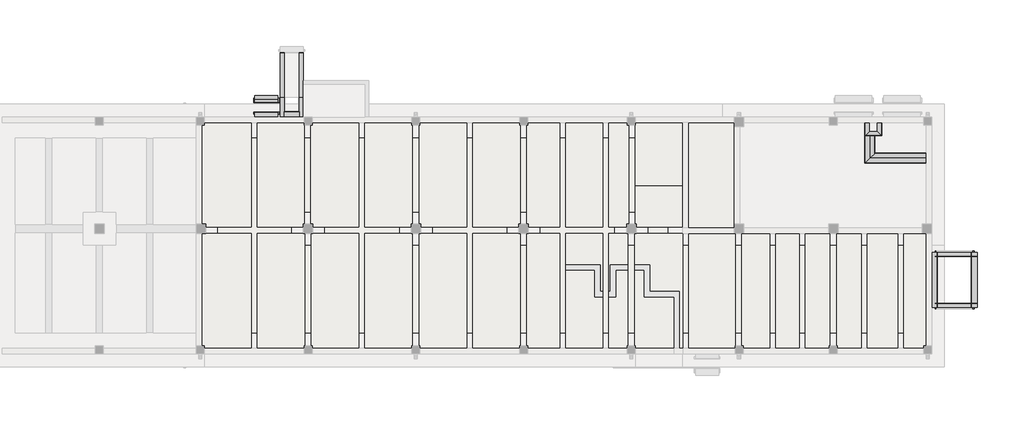
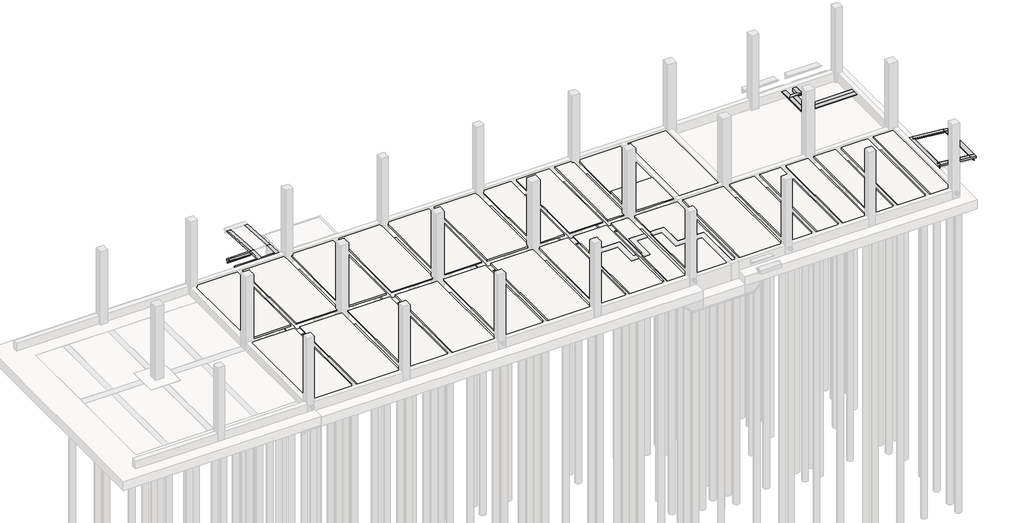
# One storey, part 2 of 7: 20 proxies, 4 slabs.
"""IFC4 building model written with IfcOpenShell, lengths in millimetres."""

from ifc_helpers import new_model, si_unit, frame, origin, place, context, project, spatial, polyline, outline, extrude, faceted_brep, element, save

model = new_model("IFC4")

# Units and contexts
model_context = context("Model", 3, world=origin())
ifc_project = project(units=[si_unit("LENGTHUNIT", "METRE", prefix="MILLI")], contexts=[model_context])

# Site, building, storey
site = spatial("IfcSite", under=ifc_project)
building = spatial("IfcBuilding", under=site)
storey = spatial("IfcBuildingStorey", under=building, Name="H.P.P", Elevation=4500.0)

# Proxies
placement = place(None, origin())
element("IfcBuildingElementProxy", 1, Name="H_SF_AR_B08_Ramp_T150_FrontEdge", ObjectType="H_SF_AR_B08_Ramp_T150_FrontEdge", at=placement, inside=storey, context=model_context, shape_type="Brep", body=[
    faceted_brep([(69312.0, -9750.0, 4500.0), (69312.0, -9750.0, 4650.0), (69700.0, -9750.0, 4650.0), (69699.3198779, -9750.0, 4649.3198779), (69562.2761194, -9750.0, 4512.2761194), (69550.0, -9750.0, 4500.0), (69312.0, -13850.0, 4650.0), (69312.0, -13850.0, 4500.0), (69550.0, -13850.0, 4500.0), (69562.2761194, -13850.0, 4512.2761194), (69699.3198779, -13850.0, 4649.3198779), (69700.0, -13850.0, 4650.0)], [[[0, 1, 2, 3, 4, 5]], [[6, 7, 8, 9, 10, 11]], [[1, 0, 7, 6]], [[8, 5, 4, 3, 2, 11, 10, 9]], [[0, 5, 8, 7]], [[2, 1, 6, 11]]]),
])
element("IfcBuildingElementProxy", 2, Name="H_SF_AR_B08_Ramp_T150_SideEdge", ObjectType="H_SF_AR_B08_Ramp_T150_SideEdge", at=placement, inside=storey, context=model_context, shape_type="Brep", body=[
    faceted_brep([(72700.0, -9750.0, 4198.5037314), (72700.0, -9750.0, 4349.2518657), (72700.0, -10050.0, 4349.2518657), (72700.0, -9900.7444215, 4199.2518657), (72700.0, -9900.0, 4198.5037314), (72692.5186568, -9750.0, 4199.2518657), (72423.0534826, -9750.0, 4226.1983831), (69562.2761194, -9750.0, 4512.2761194), (69699.3198779, -9750.0, 4649.3198779), (69700.0, -9750.0, 4649.2518657), (72250.0, -9750.0, 4394.2518657), (72256.3868159, -9750.0, 4393.6131841), (69699.3198779, -10050.0, 4649.3198779), (69700.0, -10050.0, 4649.2518657), (72250.0, -10050.0, 4394.2518657), (72255.5555556, -10050.0, 4393.6963101), (72256.3868159, -10050.0, 4393.6131841), (69562.2761194, -9900.0, 4512.2761194), (69626.5585541, -9900.0, 4505.847876), (72345.3173228, -9900.0, 4233.9719991), (72423.0534826, -9900.0, 4226.1983831), (72423.8847429, -9900.0, 4226.1152571), (72692.5186568, -9900.0, 4199.2518657)], [[[0, 1, 2, 3, 4]], [[1, 0, 5, 6, 7, 8, 9, 10, 11]], [[2, 1, 11, 10, 9, 8, 12, 13, 14, 15, 16]], [[4, 3, 2, 16, 15, 14, 13, 12, 17, 18, 19, 20, 21, 22]], [[0, 4, 22, 21, 20, 19, 18, 17, 7, 6, 5]], [[8, 7, 17, 12]]]),
    faceted_brep([(72700.0, -13850.0, 4349.2518657), (72700.0, -13850.0, 4198.5037314), (72700.0, -13700.0, 4198.5037314), (72700.0, -13699.2555785, 4199.2518657), (72700.0, -13550.0, 4349.2518657), (72256.3868159, -13850.0, 4393.6131841), (72250.0, -13850.0, 4394.2518657), (69700.0, -13850.0, 4649.2518657), (69699.3198779, -13850.0, 4649.3198779), (69562.2761194, -13850.0, 4512.2761194), (72423.0534826, -13850.0, 4226.1983831), (72692.5186568, -13850.0, 4199.2518657), (72256.3868159, -13550.0, 4393.6131841), (72255.5555556, -13550.0, 4393.6963101), (72250.0, -13550.0, 4394.2518657), (69700.0, -13550.0, 4649.2518657), (69699.3198779, -13550.0, 4649.3198779), (72692.5186568, -13700.0, 4199.2518657), (72423.8847429, -13700.0, 4226.1152571), (72423.0534826, -13700.0, 4226.1983831), (72345.3173228, -13700.0, 4233.9719991), (69626.5585541, -13700.0, 4505.847876), (69562.2761194, -13700.0, 4512.2761194)], [[[0, 1, 2, 3, 4]], [[1, 0, 5, 6, 7, 8, 9, 10, 11]], [[0, 4, 12, 13, 14, 15, 16, 8, 7, 6, 5]], [[4, 3, 2, 17, 18, 19, 20, 21, 22, 16, 15, 14, 13, 12]], [[2, 1, 11, 10, 9, 22, 21, 20, 19, 18, 17]], [[9, 8, 16, 22]]]),
])
element("IfcBuildingElementProxy", 3, Name="H_SF_AR_B08_Ramp_T150_FrontEdge(SLOPE)", ObjectType="H_SF_AR_B08_Ramp_T150_FrontEdge(SLOPE)", at=placement, inside=storey, context=model_context, shape_type="Brep", body=[
    faceted_brep([(72450.0, -13850.0, 4199.2518657), (72692.5186568, -13850.0, 4199.2518657), (72423.0534826, -13850.0, 4226.1983831), (72692.5186568, -9750.0, 4199.2518657), (72450.0, -9750.0, 4199.2518657), (72423.0534826, -9750.0, 4226.1983831), (72700.0, -13699.2555785, 4199.2518657), (72700.0, -9900.7444215, 4199.2518657), (72700.0, -10050.0, 4349.2518657), (72700.0, -13550.0, 4349.2518657), (72692.5186568, -9900.0, 4199.2518657), (72692.5186568, -13700.0, 4199.2518657), (72423.0534826, -13700.0, 4226.1983831), (72255.5555556, -13550.0, 4393.6963101), (72255.5555556, -10050.0, 4393.6963101), (72423.0534826, -9900.0, 4226.1983831)], [[[0, 1, 2]], [[3, 4, 5]], [[6, 7, 8, 9]], [[0, 4, 3, 10, 7, 6, 11, 1]], [[4, 0, 2, 12, 13, 14, 15, 5]], [[9, 8, 14, 13]], [[10, 15, 14, 8, 7]], [[15, 10, 3, 5]], [[12, 11, 6, 9, 13]], [[11, 12, 2, 1]]]),
])
element("IfcBuildingElementProxy", 4, Name="H_SF_AR_S18_Lean_T50_150X150", ObjectType="H_SF_AR_S18_Lean_T50_150X150", at=placement, inside=storey, context=model_context, shape_type="Brep", body=[
    faceted_brep([(69550.0, -13950.0, 4500.0), (69550.0, -13950.0, 4450.0), (69570.7106781, -13950.0, 4450.0), (69580.8773013, -13950.0, 4460.1666231), (69626.5585541, -13950.0, 4505.847876), (69562.2761194, -13950.0, 4512.2761194), (69550.0, -9650.0, 4450.0), (69550.0, -9650.0, 4500.0), (69562.2761194, -9650.0, 4512.2761194), (69626.5585541, -9650.0, 4505.847876), (69580.8773013, -9650.0, 4460.1666231), (69570.7106781, -9650.0, 4450.0), (69562.2761194, -13850.0, 4512.2761194), (69562.2761194, -13700.0, 4512.2761194), (69699.3198779, -13550.0, 4649.3198779), (69699.3198779, -13850.0, 4649.3198779), (69700.0, -13850.0, 4650.0), (69700.0, -9750.0, 4650.0), (69699.3198779, -9750.0, 4649.3198779), (69699.3198779, -10050.0, 4649.3198779), (69562.2761194, -9900.0, 4512.2761194), (69562.2761194, -9750.0, 4512.2761194), (69626.5585541, -9900.0, 4505.847876), (69720.7106781, -10003.0533515, 4600.0), (69720.7106781, -10050.0, 4600.0), (69717.9210597, -10050.0, 4597.2103816), (69717.9210597, -13550.0, 4597.2103816), (69720.7106781, -13550.0, 4600.0), (69720.7106781, -13596.9466485, 4600.0), (69626.5585541, -13700.0, 4505.847876), (69700.0, -13550.0, 4600.0), (69700.0, -13599.007438, 4600.0), (69700.0, -10050.0, 4600.0), (69700.0, -10000.992562, 4600.0), (69700.0, -13550.0, 4599.0024876), (69700.0, -10050.0, 4599.0024876), (69700.0, -10050.0, 4649.2518657), (69700.0, -9750.0, 4649.2518657), (69700.0, -13850.0, 4649.2518657), (69700.0, -13550.0, 4649.2518657)], [[[0, 1, 2, 3, 4, 5]], [[6, 7, 8, 9, 10, 11]], [[7, 0, 5, 12, 13, 14, 15, 16, 17, 18, 19, 20, 21, 8]], [[1, 0, 7, 6]], [[2, 1, 6, 11]], [[2, 11, 10, 9, 22, 23, 24, 25, 26, 27, 28, 29, 4, 3]], [[27, 30, 31, 28]], [[32, 24, 23, 33]], [[34, 35, 32, 33, 36, 37, 17, 16, 38, 39, 31, 30]], [[35, 34, 26, 25]], [[34, 30, 27, 26]], [[32, 35, 25, 24]], [[36, 19, 18, 37]], [[19, 36, 33, 23, 22, 20]], [[14, 39, 38, 15]], [[39, 14, 13, 29, 28, 31]], [[16, 15, 38]], [[5, 4, 29, 13, 12]], [[18, 17, 37]], [[9, 8, 21, 20, 22]]]),
])
element("IfcBuildingElementProxy", 5, Name="H_SF_AR_S18_Lean_T50_200X200", ObjectType="H_SF_AR_S18_Lean_T50_200X200", at=placement, inside=storey, context=model_context, shape_type="Brep", body=[
    faceted_brep([(72450.0, -9650.0, 4200.0), (72450.0, -9650.0, 4150.0), (72429.2893219, -9650.0, 4150.0), (72401.1499651, -9650.0, 4178.1393567), (72345.3173228, -9650.0, 4233.9719991), (72423.8847429, -9650.0, 4226.1152571), (72450.0, -13950.0, 4150.0), (72450.0, -13950.0, 4200.0), (72423.8847429, -13950.0, 4226.1152571), (72345.3173228, -13950.0, 4233.9719991), (72401.1499651, -13950.0, 4178.1393567), (72429.2893219, -13950.0, 4150.0), (72423.8847429, -9900.0, 4226.1152571), (72256.3868159, -10050.0, 4393.6131841), (72256.3868159, -9750.0, 4393.6131841), (72250.0, -9750.0, 4400.0), (72250.0, -13850.0, 4400.0), (72256.3868159, -13850.0, 4393.6131841), (72256.3868159, -13550.0, 4393.6131841), (72423.8847429, -13700.0, 4226.1152571), (72345.3173228, -13700.0, 4233.9719991), (72229.2893219, -13596.0930416, 4350.0), (72229.2893219, -13550.0, 4350.0), (72229.2893219, -10050.0, 4350.0), (72229.2893219, -10003.9069584, 4350.0), (72345.3173228, -9900.0, 4233.9719991), (72250.0, -13594.0322521, 4350.0), (72250.0, -13550.0, 4350.0), (72250.0, -10050.0, 4350.0), (72250.0, -10005.9677479, 4350.0), (72250.0, -9750.0, 4394.2518657), (72250.0, -10050.0, 4394.2518657), (72250.0, -13550.0, 4394.2518657), (72250.0, -13850.0, 4394.2518657)], [[[0, 1, 2, 3, 4, 5]], [[6, 7, 8, 9, 10, 11]], [[7, 0, 5, 12, 13, 14, 15, 16, 17, 18, 19, 8]], [[1, 0, 7, 6]], [[2, 1, 6, 11]], [[2, 11, 10, 9, 20, 21, 22, 23, 24, 25, 4, 3]], [[24, 23, 22, 21, 26, 27, 28, 29]], [[16, 15, 30, 31, 29, 28, 27, 26, 32, 33]], [[13, 31, 30, 14]], [[31, 13, 12, 25, 24, 29]], [[32, 18, 17, 33]], [[18, 32, 26, 21, 20, 19]], [[17, 16, 33]], [[9, 8, 19, 20]], [[15, 14, 30]], [[5, 4, 25, 12]]]),
])
element("IfcBuildingElementProxy", 6, Name="H_SF_AR_S18_Lean_T50_150X150", ObjectType="H_SF_AR_S18_Lean_T50_150X150", at=placement, inside=storey, context=model_context, shape_type="Brep", body=[
    faceted_brep([(72401.1499651, -13550.0, 4379.1368692), (72401.1499651, -13700.0, 4228.3887349), (72401.1499651, -13700.0, 4178.1393567), (72401.1499651, -13679.2893219, 4178.1393567), (72401.1499651, -13529.2893219, 4328.8874911), (72401.1499651, -13550.0, 4328.8874911), (69580.8773013, -13550.0, 4661.1641356), (69580.8773013, -13550.0, 4610.9147575), (69580.8773013, -13529.2893219, 4610.9147575), (69580.8773013, -13679.2893219, 4460.1666231), (69580.8773013, -13700.0, 4460.1666231), (69580.8773013, -13700.0, 4510.4160012)], [[[0, 1, 2, 3, 4, 5]], [[6, 7, 8, 9, 10, 11]], [[1, 0, 6, 11]], [[2, 1, 11, 10]], [[3, 2, 10, 9]], [[4, 3, 9, 8]], [[5, 4, 8, 7]], [[0, 5, 7, 6]]]),
])
element("IfcBuildingElementProxy", 7, Name="H_SF_AR_S18_Lean_T50_150X150", ObjectType="H_SF_AR_S18_Lean_T50_150X150", at=placement, inside=storey, context=model_context, shape_type="Brep", body=[
    faceted_brep([(69580.8773013, -10050.0, 4661.1641356), (69580.8773013, -9900.0, 4510.4160012), (69580.8773013, -9900.0, 4460.1666231), (69580.8773013, -9920.7106781, 4460.1666231), (69580.8773013, -10070.7106781, 4610.9147575), (69580.8773013, -10050.0, 4610.9147575), (72401.1499651, -10050.0, 4379.1368692), (72401.1499651, -10050.0, 4328.8874911), (72401.1499651, -10070.7106781, 4328.8874911), (72401.1499651, -9920.7106781, 4178.1393567), (72401.1499651, -9900.0, 4178.1393567), (72401.1499651, -9900.0, 4228.3887349)], [[[0, 1, 2, 3, 4, 5]], [[6, 7, 8, 9, 10, 11]], [[1, 0, 6, 11]], [[2, 1, 11, 10]], [[3, 2, 10, 9]], [[4, 3, 9, 8]], [[5, 4, 8, 7]], [[0, 5, 7, 6]]]),
])
element("IfcBuildingElementProxy", 8, Name="H_SF_AR_B08_Stoop_T150_FrontEdge", ObjectType="H_SF_AR_B08_Stoop_T150_FrontEdge", at=placement, inside=storey, context=model_context, shape_type="SweptSolid", body=[
    extrude(outline(polyline([(312.0000074, 4480.0), (312.0000074, 4630.0), (662.0000074, 4630.0), (512.0000074, 4480.0), (312.0000074, 4480.0)])), frame((19050.0, 0.0, 0.0), z_axis=(1.0, 0.0, 0.0), x_axis=(0.0, 1.0, 0.0)), (0.0, 0.0, 1.0), 1700.0),
])
element("IfcBuildingElementProxy", 9, Name="H_SF_AR_B08_Stoop_T150_FrontEdge_500x300", ObjectType="H_SF_AR_B08_Stoop_T150_FrontEdge_500x300", at=placement, inside=storey, context=model_context, shape_type="SweptSolid", body=[
    extrude(outline(polyline([(1700.0, 4330.0), (1400.0, 4630.0), (1600.0, 4630.0), (1600.0, 4515.0), (1900.0, 4515.0), (1900.0, 4330.0), (1700.0, 4330.0)])), frame((19050.0, 0.0, 0.0), z_axis=(1.0, 0.0, 0.0), x_axis=(0.0, 1.0, 0.0)), (0.0, 0.0, 1.0), 1700.0),
])
element("IfcBuildingElementProxy", 10, Name="H_SF_AR_S18_Lean_T50_300X300", ObjectType="H_SF_AR_S18_Lean_T50_300X300", at=placement, inside=storey, context=model_context, shape_type="SweptSolid", body=[
    extrude(outline(polyline([(1700.0, 4330.0), (1700.0, 4280.0), (1679.2893219, 4280.0), (1379.2893219, 4580.0), (1400.0, 4580.0), (1400.0, 4630.0), (1700.0, 4330.0)])), frame((18950.0, 0.0, 0.0), z_axis=(1.0, 0.0, 0.0), x_axis=(0.0, 1.0, 0.0)), (0.0, 0.0, 1.0), 1900.0),
])
element("IfcBuildingElementProxy", 11, Name="H_SF_AR_S18_Lean_T50_150X150", ObjectType="H_SF_AR_S18_Lean_T50_150X150", at=placement, inside=storey, context=model_context, shape_type="SweptSolid", body=[
    extrude(outline(polyline([(512.0000074, 4430.0), (512.0000074, 4480.0), (662.0000074, 4630.0), (662.0000074, 4580.0), (682.7106855, 4580.0), (532.7106855, 4430.0), (512.0000074, 4430.0)])), frame((18950.0, 0.0, 0.0), z_axis=(1.0, 0.0, 0.0), x_axis=(0.0, 1.0, 0.0)), (0.0, 0.0, 1.0), 1900.0),
])
element("IfcBuildingElementProxy", 12, Name="H_SF_AR_B08_Ramp_T150_FrontEdge", ObjectType="H_SF_AR_B08_Ramp_T150_FrontEdge", at=placement, inside=storey, context=model_context, shape_type="Brep", body=[
    faceted_brep([(21088.0, 312.0, 4450.0), (22488.0, 312.0, 4450.0), (22338.0, 312.0, 4600.0), (21238.0, 312.0, 4600.0), (22338.0, 700.0, 4600.0), (21238.0, 700.0, 4600.0), (22488.0, 550.0, 4450.0), (21088.0, 550.0, 4450.0)], [[[0, 1, 2, 3]], [[3, 2, 4, 5]], [[5, 4, 6, 7]], [[1, 0, 7, 6]], [[0, 3, 5, 7]], [[2, 1, 6, 4]]]),
])
element("IfcBuildingElementProxy", 13, Name="H_SF_AR_B08_Ramp_T150_SideEdge", ObjectType="H_SF_AR_B08_Ramp_T150_SideEdge", at=placement, inside=storey, context=model_context, shape_type="Brep", body=[
    faceted_brep([(20938.0, 1800.0, 4600.0), (21238.0, 1800.0, 4600.0), (21237.6670362, 1800.0, 4599.6670362), (21088.0, 1800.0, 4450.0), (20938.0, 1800.0, 4450.0), (20938.0, 1800.0, 4599.6670362), (20938.0, 312.0, 4600.0), (20938.0, 312.0, 4450.0), (21088.0, 312.0, 4450.0), (21238.0, 312.0, 4600.0), (21238.0, 700.0, 4600.0), (21088.0, 550.0, 4450.0)], [[[0, 1, 2, 3, 4, 5]], [[6, 7, 8, 9]], [[7, 6, 0, 5, 4]], [[1, 0, 6, 9, 10]], [[9, 8, 11, 3, 2, 1, 10]], [[4, 3, 11, 8, 7]]]),
    faceted_brep([(20938.0, 1800.0, 4599.6670362), (20938.0, 1800.0, 4449.3340724), (21088.0, 1800.0, 4449.3340724), (21238.0, 1800.0, 4599.6670362), (20938.0, 5100.0, 4379.6670362), (20938.0, 5260.3575388, 4219.3094974), (20938.0, 5261.0710326, 4218.5960036), (20938.0, 5185.3095918, 4223.6467663), (21238.0, 5100.0, 4379.6670362), (21088.0, 5185.3095918, 4223.6467663), (21088.0, 5261.0710326, 4218.5960036)], [[[0, 1, 2, 3]], [[1, 0, 4, 5, 6, 7]], [[0, 3, 8, 4]], [[3, 2, 9, 10, 8]], [[2, 1, 7, 6, 10, 9]], [[6, 5, 4, 8, 10]]]),
    faceted_brep([(22638.0, 1800.0, 4449.3340724), (22638.0, 1800.0, 4599.6670362), (22338.0, 1800.0, 4599.6670362), (22488.0, 1800.0, 4449.3340724), (22638.0, 5185.3095918, 4223.6467663), (22638.0, 5261.0710326, 4218.5960036), (22638.0, 5260.3575388, 4219.3094974), (22638.0, 5100.0, 4379.6670362), (22338.0, 5100.0, 4379.6670362), (22488.0, 5261.0710326, 4218.5960036), (22488.0, 5185.3095918, 4223.6467663)], [[[0, 1, 2, 3]], [[1, 0, 4, 5, 6, 7]], [[2, 1, 7, 8]], [[3, 2, 8, 9, 10]], [[0, 3, 10, 9, 5, 4]], [[7, 6, 5, 9, 8]]]),
    faceted_brep([(22638.0, 312.0, 4450.0), (22638.0, 312.0, 4600.0), (22338.0, 312.0, 4600.0), (22488.0, 312.0, 4450.0), (22338.0, 1800.0, 4600.0), (22638.0, 1800.0, 4600.0), (22638.0, 1800.0, 4599.6670362), (22638.0, 1800.0, 4450.0), (22488.0, 1800.0, 4450.0), (22338.3329638, 1800.0, 4599.6670362), (22338.0, 700.0, 4600.0), (22488.0, 550.0, 4450.0)], [[[0, 1, 2, 3]], [[4, 5, 6, 7, 8, 9]], [[1, 0, 7, 6, 5]], [[2, 1, 5, 4, 10]], [[3, 2, 10, 4, 9, 8, 11]], [[0, 3, 11, 8, 7]]]),
])
element("IfcBuildingElementProxy", 14, Name="H_SF_AR_S18_Lean_T50_150X150", ObjectType="H_SF_AR_S18_Lean_T50_150X150", at=placement, inside=storey, context=model_context, shape_type="Brep", body=[
    faceted_brep([(22338.0, 700.0, 4600.0), (22488.0, 550.0, 4450.0), (22488.0, 550.0, 4400.0), (22467.2893219, 570.7106781, 4400.0), (22317.2893219, 720.7106781, 4550.0), (22338.0, 700.0, 4550.0), (21088.0, 550.0, 4450.0), (21238.0, 700.0, 4600.0), (21238.0, 700.0, 4550.0), (21258.7106781, 720.7106781, 4550.0), (21108.7106781, 570.7106781, 4400.0), (21088.0, 550.0, 4400.0)], [[[0, 1, 2, 3, 4, 5]], [[6, 7, 8, 9, 10, 11]], [[1, 0, 7, 6]], [[2, 1, 6, 11]], [[3, 2, 11, 10]], [[4, 3, 10, 9]], [[5, 4, 9, 8]], [[0, 5, 8, 7]]]),
])
element("IfcBuildingElementProxy", 15, Name="H_SF_AR_S17_SOG Edge_350x150", ObjectType="H_SF_AR_S17_SOG Edge_350x150", at=placement, inside=storey, context=model_context, shape_type="Brep", body=[
    faceted_brep([(64707.0, -2743.0, 4500.0), (64707.0, -2743.0, 4650.0), (64707.0, -1062.0, 4650.0), (64707.0, -912.0, 4500.0), (65057.0, -2393.0, 4650.0), (64907.0, -2543.0, 4500.0), (64907.0, -982.7106781, 4500.0), (64907.0, -912.0, 4500.0), (65057.0, -1062.0, 4650.0), (68888.0, -2743.0, 4650.0), (68888.0, -2743.0, 4500.0), (68888.0, -2543.0, 4500.0), (68888.0, -2393.0, 4650.0)], [[[0, 1, 2, 3]], [[4, 5, 6, 7, 8]], [[5, 0, 3, 7, 6]], [[1, 4, 8, 2]], [[9, 10, 11, 12]], [[1, 0, 10, 9]], [[4, 1, 9, 12]], [[5, 4, 12, 11]], [[0, 5, 11, 10]], [[3, 2, 8, 7]]]),
])
element("IfcBuildingElementProxy", 16, Name="H_SF_AR_S17_SOG Edge_350x150", ObjectType="H_SF_AR_S17_SOG Edge_350x150", at=placement, inside=storey, context=model_context, shape_type="Brep", body=[
    faceted_brep([(64707.0, -2743.0, 4650.0), (64707.0, -2743.0, 4500.0), (64707.0, -912.0, 4500.0), (64707.0, -1062.0, 4650.0), (64357.0, -3093.0, 4650.0), (64357.0, -1062.0, 4650.0), (64507.0, -2943.0, 4500.0), (64507.0, -912.0, 4500.0), (64507.0, -982.7106781, 4500.0), (68888.0, -2743.0, 4500.0), (68888.0, -2743.0, 4650.0), (68888.0, -3093.0, 4650.0), (68888.0, -2943.0, 4500.0)], [[[0, 1, 2, 3]], [[4, 0, 3, 5]], [[6, 4, 5, 7, 8]], [[1, 6, 8, 7, 2]], [[9, 10, 11, 12]], [[1, 0, 10, 9]], [[0, 4, 11, 10]], [[4, 6, 12, 11]], [[6, 1, 9, 12]], [[3, 2, 7, 5]]]),
])
element("IfcBuildingElementProxy", 17, Name="H_SF_AR_S17_SOG Edge_300x300", ObjectType="H_SF_AR_S17_SOG Edge_300x300", at=placement, inside=storey, context=model_context, shape_type="Brep", body=[
    faceted_brep([(64657.0, -112.0, 4350.0), (64357.0, -112.0, 4650.0), (64657.0, -112.0, 4650.0), (64357.0, -1062.0, 4650.0), (64657.0, -762.0, 4650.0), (64657.0, -762.0, 4350.0), (64507.0, -912.0, 4500.0), (65257.0, -762.0, 4350.0), (65557.0, -1062.0, 4650.0), (65057.0, -1062.0, 4650.0), (64707.0, -1062.0, 4650.0), (65257.0, -762.0, 4650.0), (65557.0, -112.0, 4650.0), (65257.0, -112.0, 4350.0), (65257.0, -112.0, 4650.0)], [[[0, 1, 2]], [[1, 3, 4, 2]], [[1, 0, 5, 6, 3]], [[3, 6, 5, 7, 8, 9, 10]], [[3, 10, 9, 8, 11, 4]], [[12, 13, 14]], [[8, 7, 13, 12]], [[8, 12, 14, 11]], [[7, 11, 14, 13]], [[11, 7, 5, 4]], [[4, 5, 0, 2]]]),
])
element("IfcBuildingElementProxy", 18, Name="H_SF_AR_S18_Lean_T50_150X150", ObjectType="H_SF_AR_S18_Lean_T50_150X150", at=placement, inside=storey, context=model_context, shape_type="Brep", body=[
    faceted_brep([(64357.0, -3093.0, 4650.0), (64507.0, -2943.0, 4500.0), (64507.0, -982.7106781, 4500.0), (64407.0, -1082.7106781, 4600.0), (64407.0, -1062.0, 4600.0), (64357.0, -1062.0, 4650.0), (64507.0, -2943.0, 4450.0), (64507.0, -932.7106781, 4450.0), (64486.2893219, -2963.7106781, 4450.0), (64486.2893219, -932.7106781, 4450.0), (64336.2893219, -3113.7106781, 4600.0), (64336.2893219, -1082.7106781, 4600.0), (64357.0, -3093.0, 4600.0), (64357.0, -1082.7106781, 4600.0), (64357.0, -1062.0, 4600.0), (68900.0, -2943.0, 4500.0), (68900.0, -3093.0, 4650.0), (68900.0, -3093.0, 4600.0), (68900.0, -3113.7106781, 4600.0), (68900.0, -2963.7106781, 4450.0), (68900.0, -2943.0, 4450.0)], [[[0, 1, 2, 3, 4, 5]], [[1, 6, 7, 2]], [[6, 8, 9, 7]], [[8, 10, 11, 9]], [[10, 12, 13, 11]], [[12, 0, 5, 14, 13]], [[15, 16, 17, 18, 19, 20]], [[1, 0, 16, 15]], [[6, 1, 15, 20]], [[8, 6, 20, 19]], [[10, 8, 19, 18]], [[12, 10, 18, 17]], [[0, 12, 17, 16]], [[13, 3, 2, 7, 9, 11]], [[3, 13, 14, 4]], [[4, 14, 5]]]),
])
element("IfcBuildingElementProxy", 19, Name="H_SF_AR_S18_Lean_T50_150X150", ObjectType="H_SF_AR_S18_Lean_T50_150X150", at=placement, inside=storey, context=model_context, shape_type="Brep", body=[
    faceted_brep([(64907.0, -2543.0, 4500.0), (65057.0, -2393.0, 4650.0), (65057.0, -1062.0, 4650.0), (65007.0, -1062.0, 4600.0), (65007.0, -1082.7106781, 4600.0), (64907.0, -982.7106781, 4500.0), (64907.0, -2543.0, 4450.0), (64907.0, -932.7106781, 4450.0), (64927.7106781, -2522.2893219, 4450.0), (64927.7106781, -932.7106781, 4450.0), (65077.7106781, -2372.2893219, 4600.0), (65077.7106781, -1082.7106781, 4600.0), (65057.0, -2393.0, 4600.0), (65057.0, -1082.7106781, 4600.0), (65057.0, -1062.0, 4600.0), (68900.0, -2393.0, 4650.0), (68900.0, -2543.0, 4500.0), (68900.0, -2543.0, 4450.0), (68900.0, -2522.2893219, 4450.0), (68900.0, -2372.2893219, 4600.0), (68900.0, -2393.0, 4600.0)], [[[0, 1, 2, 3, 4, 5]], [[6, 0, 5, 7]], [[8, 6, 7, 9]], [[10, 8, 9, 11]], [[12, 10, 11, 13]], [[1, 12, 13, 14, 2]], [[15, 16, 17, 18, 19, 20]], [[1, 0, 16, 15]], [[0, 6, 17, 16]], [[6, 8, 18, 17]], [[8, 10, 19, 18]], [[10, 12, 20, 19]], [[12, 1, 15, 20]], [[4, 13, 11, 9, 7, 5]], [[13, 4, 3, 14]], [[14, 3, 2]]]),
])
element("IfcBuildingElementProxy", 20, Name="H_SF_AR_S18_Lean_T50_300X300", ObjectType="H_SF_AR_S18_Lean_T50_300X300", at=placement, inside=storey, context=model_context, shape_type="Brep", body=[
    faceted_brep([(64357.0, -100.0, 4650.0), (64657.0, -100.0, 4350.0), (64657.0, -100.0, 4300.0), (64636.2893219, -100.0, 4300.0), (64336.2893219, -100.0, 4600.0), (64357.0, -100.0, 4600.0), (64357.0, -1062.0, 4650.0), (64407.0, -1062.0, 4600.0), (64407.0, -1082.7106781, 4600.0), (64507.0, -982.7106781, 4500.0), (64507.0, -912.0, 4500.0), (64657.0, -762.0, 4350.0), (64657.0, -762.0, 4300.0), (64636.2893219, -782.7106781, 4300.0), (64486.2893219, -932.7106781, 4450.0), (64336.2893219, -1082.7106781, 4600.0), (64357.0, -1062.0, 4600.0), (65557.0, -1062.0, 4650.0), (65257.0, -762.0, 4350.0), (64707.0, -912.0, 4500.0), (64907.0, -912.0, 4500.0), (65057.0, -1062.0, 4650.0), (65257.0, -762.0, 4300.0), (65277.7106781, -782.7106781, 4300.0), (65577.7106781, -1082.7106781, 4600.0), (65077.7106781, -1082.7106781, 4600.0), (65057.0, -1082.7106781, 4600.0), (65007.0, -1082.7106781, 4600.0), (64907.0, -982.7106781, 4500.0), (64357.0, -1082.7106781, 4600.0), (65557.0, -1062.0, 4600.0), (65057.0, -1062.0, 4600.0), (65007.0, -1062.0, 4600.0), (65257.0, -100.0, 4350.0), (65557.0, -100.0, 4650.0), (65557.0, -100.0, 4600.0), (65577.7106781, -100.0, 4600.0), (65277.7106781, -100.0, 4300.0), (65257.0, -100.0, 4300.0)], [[[0, 1, 2, 3, 4, 5]], [[1, 0, 6, 7, 8, 9, 10, 11]], [[11, 12, 2, 1]], [[12, 13, 3, 2]], [[13, 14, 15, 4, 3]], [[15, 16, 5, 4]], [[16, 6, 0, 5]], [[17, 18, 11, 10, 19, 20, 21]], [[12, 11, 18, 22]], [[13, 12, 22, 23]], [[15, 14, 13, 23, 24, 25, 26, 27, 28, 9, 8, 29]], [[16, 15, 29, 8, 7]], [[24, 30, 31, 32, 27, 26, 25]], [[6, 16, 7]], [[30, 17, 21, 32, 31]], [[33, 34, 35, 36, 37, 38]], [[18, 17, 34, 33]], [[22, 18, 33, 38]], [[23, 22, 38, 37]], [[24, 23, 37, 36]], [[30, 24, 36, 35]], [[17, 30, 35, 34]], [[10, 9, 28, 20, 19]], [[20, 28, 27, 32, 21]]]),
])

# Slabs
element("IfcSlab", 21, ObjectType="H_FL_AR_B07_Ground Insulation_T110", at=placement, inside=storey, context=model_context, shape_type="SweptSolid", body=[
    extrude(outline(polyline([(15100.0, -8350.0), (18775.0, -8350.0), (18775.0, -16900.0), (15300.0, -16900.0), (15300.0, -16700.0), (15100.0, -16700.0), (15100.0, -8350.0)])), frame((0.0, 0.0, 4540.0), z_axis=(0.0, 0.0, 1.0), x_axis=(1.0, 0.0, 0.0)), (0.0, 0.0, 1.0), 110.0),
    extrude(outline(polyline([(15400.0000001, -7850.0), (15400.0000001, -7650.0), (15100.0, -7650.0), (15100.0, -300.0), (15300.0, -300.0), (15300.0, -100.0), (18775.0, -100.0), (18775.0, -7850.0), (15400.0000001, -7850.0)])), frame((0.0, 0.0, 4540.0), z_axis=(0.0, 0.0, 1.0), x_axis=(1.0, 0.0, 0.0)), (0.0, 0.0, 1.0), 110.0),
    extrude(outline(polyline([(22750.0, -8350.0), (22750.0, -16700.0), (22700.0, -16700.0), (22700.0, -16900.0), (19225.0, -16900.0), (19225.0, -8350.0), (22750.0, -8350.0)])), frame((0.0, 0.0, 4540.0), z_axis=(0.0, 0.0, 1.0), x_axis=(1.0, 0.0, 0.0)), (0.0, 0.0, 1.0), 110.0),
    extrude(outline(polyline([(22650.0000003, -7850.0), (19225.0, -7850.0), (19225.0, -100.0), (22700.0, -100.0), (22700.0, -7650.0), (22650.0000003, -7650.0), (22650.0000003, -7850.0)])), frame((0.0, 0.0, 4540.0), z_axis=(0.0, 0.0, 1.0), x_axis=(1.0, 0.0, 0.0)), (0.0, 0.0, 1.0), 110.0),
    extrude(outline(polyline([(23250.0, -8350.0), (26775.0, -8350.0), (26775.0, -16900.0), (23300.0, -16900.0), (23300.0, -16700.0), (23250.0, -16700.0), (23250.0, -8350.0)])), frame((0.0, 0.0, 4540.0), z_axis=(0.0, 0.0, 1.0), x_axis=(1.0, 0.0, 0.0)), (0.0, 0.0, 1.0), 110.0),
    extrude(outline(polyline([(23350.0000003, -7850.0), (23350.0000003, -7650.0), (23200.0, -7650.0), (23200.0, -300.0), (23300.0, -300.0), (23300.0, -100.0), (26775.0, -100.0), (26775.0, -7850.0), (23350.0000003, -7850.0)])), frame((0.0, 0.0, 4540.0), z_axis=(0.0, 0.0, 1.0), x_axis=(1.0, 0.0, 0.0)), (0.0, 0.0, 1.0), 110.0),
    extrude(outline(polyline([(30750.0, -8350.0), (30750.0, -16700.0), (30700.0, -16700.0), (30700.0, -16900.0), (27225.0, -16900.0), (27225.0, -8350.0), (30750.0, -8350.0)])), frame((0.0, 0.0, 4540.0), z_axis=(0.0, 0.0, 1.0), x_axis=(1.0, 0.0, 0.0)), (0.0, 0.0, 1.0), 110.0),
    extrude(outline(polyline([(30650.0000002, -7850.0), (27225.0, -7850.0), (27225.0, -100.0), (30700.0, -100.0), (30700.0, -300.0), (30750.0, -300.0), (30750.0, -7650.0), (30650.0000002, -7650.0), (30650.0000002, -7850.0)])), frame((0.0, 0.0, 4540.0), z_axis=(0.0, 0.0, 1.0), x_axis=(1.0, 0.0, 0.0)), (0.0, 0.0, 1.0), 110.0),
    extrude(outline(polyline([(31250.0, -8350.0), (34775.0, -8350.0), (34775.0, -16900.0), (31300.0, -16900.0), (31300.0, -16700.0), (31250.0, -16700.0), (31250.0, -8350.0)])), frame((0.0, 0.0, 4540.0), z_axis=(0.0, 0.0, 1.0), x_axis=(1.0, 0.0, 0.0)), (0.0, 0.0, 1.0), 110.0),
    extrude(outline(polyline([(31350.0000002, -7850.0), (31350.0000002, -7650.0), (31250.0, -7650.0), (31250.0, -300.0), (31300.0, -300.0), (31300.0, -100.0), (34775.0, -100.0), (34775.0, -7850.0), (31350.0000002, -7850.0)])), frame((0.0, 0.0, 4540.0), z_axis=(0.0, 0.0, 1.0), x_axis=(1.0, 0.0, 0.0)), (0.0, 0.0, 1.0), 110.0),
    extrude(outline(polyline([(38750.0, -8350.0), (38750.0, -16700.0), (38700.0, -16700.0), (38700.0, -16900.0), (35225.0, -16900.0), (35225.0, -8350.0), (38750.0, -8350.0)])), frame((0.0, 0.0, 4540.0), z_axis=(0.0, 0.0, 1.0), x_axis=(1.0, 0.0, 0.0)), (0.0, 0.0, 1.0), 110.0),
    extrude(outline(polyline([(38650.0000001, -7850.0), (35225.0, -7850.0), (35225.0, -100.0), (38700.0, -100.0), (38700.0, -300.0), (38750.0, -300.0), (38750.0, -7650.0), (38650.0000001, -7650.0), (38650.0000001, -7850.0)])), frame((0.0, 0.0, 4540.0), z_axis=(0.0, 0.0, 1.0), x_axis=(1.0, 0.0, 0.0)), (0.0, 0.0, 1.0), 110.0),
    extrude(outline(polyline([(39250.0, -8350.0), (41675.0, -8350.0), (41675.0, -16900.0), (39300.0, -16900.0), (39300.0, -16700.0), (39250.0, -16700.0), (39250.0, -8350.0)])), frame((0.0, 0.0, 4540.0), z_axis=(0.0, 0.0, 1.0), x_axis=(1.0, 0.0, 0.0)), (0.0, 0.0, 1.0), 110.0),
    extrude(outline(polyline([(39350.0000001, -7850.0), (39350.0000001, -7650.0), (39250.0, -7650.0), (39250.0, -300.0), (39300.0, -300.0), (39300.0, -100.0), (41675.0, -100.0), (41675.0, -7850.0), (39350.0000001, -7850.0)])), frame((0.0, 0.0, 4540.0), z_axis=(0.0, 0.0, 1.0), x_axis=(1.0, 0.0, 0.0)), (0.0, 0.0, 1.0), 110.0),
    extrude(outline(polyline([(44875.0, -100.0), (44875.0, -7850.0), (42125.0, -7850.0), (42125.0, -100.0), (44875.0, -100.0)])), frame((0.0, 0.0, 4540.0), z_axis=(0.0, 0.0, 1.0), x_axis=(1.0, 0.0, 0.0)), (0.0, 0.0, 1.0), 110.0),
    extrude(outline(polyline([(44875.0, -8350.0), (44875.0, -12675.0), (44675.0, -12675.0), (44675.0, -10675.0), (42125.0, -10675.0), (42125.0, -8350.0), (44875.0, -8350.0)])), frame((0.0, 0.0, 4540.0), z_axis=(0.0, 0.0, 1.0), x_axis=(1.0, 0.0, 0.0)), (0.0, 0.0, 1.0), 110.0),
    extrude(outline(polyline([(45325.0, -12675.0), (45325.0, -8350.0), (46750.0, -8350.0), (46750.0, -10675.0), (45425.0, -10675.0), (45425.0, -12675.0), (45325.0, -12675.0)])), frame((0.0, 0.0, 4540.0), z_axis=(0.0, 0.0, 1.0), x_axis=(1.0, 0.0, 0.0)), (0.0, 0.0, 1.0), 110.0),
    extrude(outline(polyline([(50825.0, -4825.0), (50825.0, -7850.0), (47349.9999999, -7850.0), (47349.9999999, -7650.0), (47300.0, -7650.0), (47300.0, -4825.0), (50825.0, -4825.0)])), frame((0.0, 0.0, 4540.0), z_axis=(0.0, 0.0, 1.0), x_axis=(1.0, 0.0, 0.0)), (0.0, 0.0, 1.0), 110.0),
    extrude(outline(polyline([(54700.0, -8350.0), (54700.0, -16900.0), (51275.0, -16900.0), (51275.0, -8350.0), (54700.0, -8350.0)])), frame((0.0, 0.0, 4540.0), z_axis=(0.0, 0.0, 1.0), x_axis=(1.0, 0.0, 0.0)), (0.0, 0.0, 1.0), 110.0),
    extrude(outline(polyline([(57275.0, -16900.0), (55200.0, -16900.0), (55200.0, -8350.0), (57275.0, -8350.0), (57275.0, -16900.0)])), frame((0.0, 0.0, 4540.0), z_axis=(0.0, 0.0, 1.0), x_axis=(1.0, 0.0, 0.0)), (0.0, 0.0, 1.0), 110.0),
    extrude(outline(polyline([(59475.0, -8350.0), (59475.0, -16900.0), (57725.0, -16900.0), (57725.0, -8350.0), (59475.0, -8350.0)])), frame((0.0, 0.0, 4540.0), z_axis=(0.0, 0.0, 1.0), x_axis=(1.0, 0.0, 0.0)), (0.0, 0.0, 1.0), 110.0),
    extrude(outline(polyline([(61750.0, -16900.0), (59925.0, -16900.0), (59925.0, -8350.0), (61750.0, -8350.0), (61750.0, -16900.0)])), frame((0.0, 0.0, 4540.0), z_axis=(0.0, 0.0, 1.0), x_axis=(1.0, 0.0, 0.0)), (0.0, 0.0, 1.0), 110.0),
    extrude(outline(polyline([(64075.0, -8350.0), (64075.0, -16900.0), (62250.0, -16900.0), (62250.0, -8350.0), (64075.0, -8350.0)])), frame((0.0, 0.0, 4540.0), z_axis=(0.0, 0.0, 1.0), x_axis=(1.0, 0.0, 0.0)), (0.0, 0.0, 1.0), 110.0),
    extrude(outline(polyline([(66775.0, -8350.0), (66775.0, -16900.0), (64525.0, -16900.0), (64525.0, -8350.0), (66775.0, -8350.0)])), frame((0.0, 0.0, 4540.0), z_axis=(0.0, 0.0, 1.0), x_axis=(1.0, 0.0, 0.0)), (0.0, 0.0, 1.0), 110.0),
    extrude(outline(polyline([(68700.0, -16900.0), (67225.0, -16900.0), (67225.0, -8350.0), (68900.0, -8350.0), (68900.0, -16700.0), (68700.0, -16700.0), (68700.0, -16900.0)])), frame((0.0, 0.0, 4540.0), z_axis=(0.0, 0.0, 1.0), x_axis=(1.0, 0.0, 0.0)), (0.0, 0.0, 1.0), 110.0),
    extrude(outline(polyline([(46700.0, -100.0), (46700.0, -300.0), (46800.0, -300.0), (46800.0, -7650.0), (46649.9999999, -7650.0), (46649.9999999, -7850.0), (45325.0, -7850.0), (45325.0, -100.0), (46700.0, -100.0)])), frame((0.0, 0.0, 4540.0), z_axis=(0.0, 0.0, 1.0), x_axis=(1.0, 0.0, 0.0)), (0.0, 0.0, 1.0), 110.0),
    extrude(outline(polyline([(50575.0, -16900.0), (50575.0, -12675.0), (48375.0, -12675.0), (48375.0, -10675.0), (47250.0, -10675.0), (47250.0, -8350.0), (50825.0, -8350.0), (50825.0, -16900.0), (50575.0, -16900.0)])), frame((0.0, 0.0, 4540.0), z_axis=(0.0, 0.0, 1.0), x_axis=(1.0, 0.0, 0.0)), (0.0, 0.0, 1.0), 110.0),
])
element("IfcSlab", 22, ObjectType="H_FL_AR_B07_Ground Insulation_T110", at=placement, inside=storey, context=model_context, shape_type="SweptSolid", body=[
    extrude(outline(polyline([(50475.0, -16900.0), (47300.0, -16900.0), (47300.0, -16700.0), (47250.0, -16700.0), (47250.0, -10775.0), (48275.0, -10775.0), (48275.0, -12775.0), (50475.0, -12775.0), (50475.0, -16900.0)])), frame((0.0, 0.0, 4440.0), z_axis=(0.0, 0.0, 1.0), x_axis=(1.0, 0.0, 0.0)), (0.0, 0.0, 1.0), 110.0),
    extrude(outline(polyline([(46750.0, -10775.0), (46750.0, -16700.0), (46700.0, -16700.0), (46700.0, -16900.0), (45325.0, -16900.0), (45325.0, -12775.0), (45525.0, -12775.0), (45525.0, -10775.0), (46750.0, -10775.0)])), frame((0.0, 0.0, 4440.0), z_axis=(0.0, 0.0, 1.0), x_axis=(1.0, 0.0, 0.0)), (0.0, 0.0, 1.0), 110.0),
    extrude(outline(polyline([(44875.0, -12775.0), (44875.0, -16900.0), (42125.0, -16900.0), (42125.0, -10775.0), (44575.0, -10775.0), (44575.0, -12775.0), (44875.0, -12775.0)])), frame((0.0, 0.0, 4440.0), z_axis=(0.0, 0.0, 1.0), x_axis=(1.0, 0.0, 0.0)), (0.0, 0.0, 1.0), 110.0),
    extrude(outline(polyline([(47300.0, -4825.0), (47300.0, -100.0), (50825.0, -100.0), (50825.0, -4825.0), (47300.0, -4825.0)])), frame((0.0, 0.0, 4440.0), z_axis=(0.0, 0.0, 1.0), x_axis=(1.0, 0.0, 0.0)), (0.0, 0.0, 1.0), 110.0),
])
element("IfcSlab", 23, ObjectType="H_FL_AR_B07_Ground Insulation_T110", at=placement, inside=storey, context=model_context, shape_type="SweptSolid", body=[
    extrude(outline(polyline([(19335.0, -1250.0000001), (19335.0, -7740.0), (21750.0000003, -7740.0), (21750.0000003, -8460.0), (19335.0, -8460.0), (19335.0, -15750.0000001), (18665.0, -15750.0000001), (18665.0, -8460.0), (16300.0000001, -8460.0), (16300.0000001, -7740.0), (18665.0, -7740.0), (18665.0, -1250.0000001), (19335.0, -1250.0000001)])), frame((0.0, 0.0, 3890.0), z_axis=(0.0, 0.0, 1.0), x_axis=(1.0, 0.0, 0.0)), (0.0, 0.0, 1.0), 110.0),
    extrude(outline(polyline([(23310.0, -1250.0000001), (23310.0, -6750.0), (22590.0, -6750.0), (22590.0, -1250.0000001), (23310.0, -1250.0000001)])), frame((0.0, 0.0, 3890.0), z_axis=(0.0, 0.0, 1.0), x_axis=(1.0, 0.0, 0.0)), (0.0, 0.0, 1.0), 110.0),
    extrude(outline(polyline([(23360.0, -9250.0), (23360.0, -15750.0000001), (22640.0, -15750.0000001), (22640.0, -9250.0), (23360.0, -9250.0)])), frame((0.0, 0.0, 3890.0), z_axis=(0.0, 0.0, 1.0), x_axis=(1.0, 0.0, 0.0)), (0.0, 0.0, 1.0), 110.0),
    extrude(outline(polyline([(27335.0, -1250.0000001), (27335.0, -7740.0), (29750.0000003, -7740.0), (29750.0000003, -8460.0), (27335.0, -8460.0), (27335.0, -15750.0000001), (26665.0, -15750.0000001), (26665.0, -8460.0), (24249.9999997, -8460.0), (24249.9999997, -7740.0), (26665.0, -7740.0), (26665.0, -1250.0000001), (27335.0, -1250.0000001)])), frame((0.0, 0.0, 3890.0), z_axis=(0.0, 0.0, 1.0), x_axis=(1.0, 0.0, 0.0)), (0.0, 0.0, 1.0), 110.0),
    extrude(outline(polyline([(31359.9999999, -1250.0000001), (31359.9999999, -6750.0), (30639.9999999, -6750.0), (30639.9999999, -1250.0000001), (31359.9999999, -1250.0000001)])), frame((0.0, 0.0, 3890.0), z_axis=(0.0, 0.0, 1.0), x_axis=(1.0, 0.0, 0.0)), (0.0, 0.0, 1.0), 110.0),
    extrude(outline(polyline([(31359.9999999, -9250.0), (31359.9999999, -15750.0000001), (30639.9999999, -15750.0000001), (30639.9999999, -9250.0), (31359.9999999, -9250.0)])), frame((0.0, 0.0, 3890.0), z_axis=(0.0, 0.0, 1.0), x_axis=(1.0, 0.0, 0.0)), (0.0, 0.0, 1.0), 110.0),
    extrude(outline(polyline([(35335.0, -1250.0000001), (35335.0, -7740.0), (37750.0000003, -7740.0), (37750.0000003, -8460.0), (35335.0, -8460.0), (35335.0, -15750.0000001), (34665.0, -15750.0000001), (34665.0, -8460.0), (32250.0000002, -8460.0), (32250.0000002, -7740.0), (34665.0, -7740.0), (34665.0, -1250.0000001), (35335.0, -1250.0000001)])), frame((0.0, 0.0, 3890.0), z_axis=(0.0, 0.0, 1.0), x_axis=(1.0, 0.0, 0.0)), (0.0, 0.0, 1.0), 110.0),
    extrude(outline(polyline([(39359.9999999, -1250.0000001), (39359.9999999, -6750.0), (38639.9999999, -6750.0), (38639.9999999, -1250.0000001), (39359.9999999, -1250.0000001)])), frame((0.0, 0.0, 3890.0), z_axis=(0.0, 0.0, 1.0), x_axis=(1.0, 0.0, 0.0)), (0.0, 0.0, 1.0), 110.0),
    extrude(outline(polyline([(39359.9999999, -9250.0), (39359.9999999, -15750.0000001), (38639.9999999, -15750.0000001), (38639.9999999, -9250.0), (39359.9999999, -9250.0)])), frame((0.0, 0.0, 3890.0), z_axis=(0.0, 0.0, 1.0), x_axis=(1.0, 0.0, 0.0)), (0.0, 0.0, 1.0), 110.0),
    extrude(outline(polyline([(42235.0, -1250.0000001), (42235.0, -7740.0), (44765.0, -7740.0), (44765.0, -1250.0000001), (45435.0, -1250.0000001), (45435.0, -7740.0), (45749.9999999, -7740.0), (45749.9999999, -8460.0), (45435.0, -8460.0), (45435.0, -15750.0000001), (44765.0, -15750.0000001), (44765.0, -8460.0), (42235.0, -8460.0), (42235.0, -15750.0000001), (41565.0, -15750.0000001), (41565.0, -8460.0), (40250.0000001, -8460.0), (40250.0000001, -7740.0), (41565.0, -7740.0), (41565.0, -1250.0000001), (42235.0, -1250.0000001)])), frame((0.0, 0.0, 3890.0), z_axis=(0.0, 0.0, 1.0), x_axis=(1.0, 0.0, 0.0)), (0.0, 0.0, 1.0), 110.0),
    extrude(outline(polyline([(47409.9999996, -1250.0000001), (47409.9999996, -6750.0), (46689.9999996, -6750.0), (46689.9999996, -1250.0000001), (47409.9999996, -1250.0000001)])), frame((0.0, 0.0, 3890.0), z_axis=(0.0, 0.0, 1.0), x_axis=(1.0, 0.0, 0.0)), (0.0, 0.0, 1.0), 110.0),
    extrude(outline(polyline([(47359.9999996, -9250.0), (47359.9999996, -15750.0000001), (46639.9999996, -15750.0000001), (46639.9999996, -9250.0), (47359.9999996, -9250.0)])), frame((0.0, 0.0, 3890.0), z_axis=(0.0, 0.0, 1.0), x_axis=(1.0, 0.0, 0.0)), (0.0, 0.0, 1.0), 110.0),
    extrude(outline(polyline([(49700.0000002, -8460.0), (48249.9999999, -8460.0), (48249.9999999, -7740.0), (49700.0000002, -7740.0), (49700.0000002, -8460.0)])), frame((0.0, 0.0, 3890.0), z_axis=(0.0, 0.0, 1.0), x_axis=(1.0, 0.0, 0.0)), (0.0, 0.0, 1.0), 110.0),
    extrude(outline(polyline([(50715.0, -15750.0000001), (50715.0, -9250.0), (51385.0, -9250.0), (51385.0, -15750.0000001), (50715.0, -15750.0000001)])), frame((0.0, 0.0, 3890.0), z_axis=(0.0, 0.0, 1.0), x_axis=(1.0, 0.0, 0.0)), (0.0, 0.0, 1.0), 110.0),
    extrude(outline(polyline([(54590.0, -15750.0000001), (54590.0, -9250.0), (55310.0, -9250.0), (55310.0, -15750.0000001), (54590.0, -15750.0000001)])), frame((0.0, 0.0, 3890.0), z_axis=(0.0, 0.0, 1.0), x_axis=(1.0, 0.0, 0.0)), (0.0, 0.0, 1.0), 110.0),
    extrude(outline(polyline([(57165.0, -15750.0000001), (57165.0, -9250.0), (57835.0, -9250.0), (57835.0, -15750.0000001), (57165.0, -15750.0000001)])), frame((0.0, 0.0, 3890.0), z_axis=(0.0, 0.0, 1.0), x_axis=(1.0, 0.0, 0.0)), (0.0, 0.0, 1.0), 110.0),
    extrude(outline(polyline([(59365.0, -15750.0000001), (59365.0, -9250.0), (60035.0, -9250.0), (60035.0, -15750.0000001), (59365.0, -15750.0000001)])), frame((0.0, 0.0, 3890.0), z_axis=(0.0, 0.0, 1.0), x_axis=(1.0, 0.0, 0.0)), (0.0, 0.0, 1.0), 110.0),
    extrude(outline(polyline([(61640.0, -15750.0000001), (61640.0, -9250.0), (62360.0, -9250.0), (62360.0, -15750.0000001), (61640.0, -15750.0000001)])), frame((0.0, 0.0, 3890.0), z_axis=(0.0, 0.0, 1.0), x_axis=(1.0, 0.0, 0.0)), (0.0, 0.0, 1.0), 110.0),
    extrude(outline(polyline([(63965.0, -15750.0000001), (63965.0, -9250.0), (64635.0, -9250.0), (64635.0, -15750.0000001), (63965.0, -15750.0000001)])), frame((0.0, 0.0, 3890.0), z_axis=(0.0, 0.0, 1.0), x_axis=(1.0, 0.0, 0.0)), (0.0, 0.0, 1.0), 110.0),
    extrude(outline(polyline([(66665.0, -15750.0000001), (66665.0, -9250.0), (67335.0, -9250.0), (67335.0, -15750.0000001), (66665.0, -15750.0000001)])), frame((0.0, 0.0, 3890.0), z_axis=(0.0, 0.0, 1.0), x_axis=(1.0, 0.0, 0.0)), (0.0, 0.0, 1.0), 110.0),
])
element("IfcSlab", 24, ObjectType="H_FL_AR_B07_Ground Insulation_T110", at=placement, inside=storey, context=model_context, shape_type="SweptSolid", body=[
    extrude(outline(polyline([(54650.0, -100.0), (54650.0, -7950.0), (51225.0, -7950.0), (51225.0, -100.0), (54650.0, -100.0)])), frame((0.0, 0.0, 4490.0), z_axis=(0.0, 0.0, 1.0), x_axis=(1.0, 0.0, 0.0)), (0.0, 0.0, 1.0), 110.0),
])

save(model, "model.ifc")

# Revit data of these elements
# Type "H_SF_AR_B08_Ramp_T150_FrontEdge"
#   Type Comments = "CV-UG"
#   H_Rebar Ratio = 0.12
# Type "H_SF_AR_B08_Ramp_T150_SideEdge"
#   Type Comments = "CV-UG"
#   H_Rebar Ratio = 0.12
# Type "H_SF_AR_B08_Ramp_T150_FrontEdge(SLOPE)"
#   Type Comments = "CV-UG"
#   H_Rebar Ratio = 0.12
# Type "H_SF_AR_S18_Lean_T50_150X150"
#   Type Comments = "Lean"
# Type "H_SF_AR_S18_Lean_T50_200X200"
#   Type Comments = "Lean"
# Type "H_SF_AR_B08_Stoop_T150_FrontEdge"
#   Type Comments = "CV-UG"
#   H_Rebar Ratio = 0.12
# Type "H_SF_AR_B08_Stoop_T150_FrontEdge_500x300"
#   Type Comments = "CV-UG"
#   H_Rebar Ratio = 0.12
# Type "H_SF_AR_S18_Lean_T50_300X300"
#   Type Comments = "Lean"
# Type "H_SF_AR_S17_SOG Edge_350x150"
#   Type Comments = "CV-UG"
#   H_Rebar Ratio = 0.1
# Type "H_SF_AR_S17_SOG Edge_300x300"
#   Type Comments = "CV-UG"
#   H_Rebar Ratio = 0.1
# Type "H_FL_AR_B07_Ground Insulation_T110"
#   Keynote = ""
#   Type Comments = "Finish"
#   Description = ""
#   Function = 0
#   Layers, outside or top first: 110 mm "00_Insulation_Rigid" (function 3); 0 mm "00_P.E Film" (function 100); 0 mm "00_P.E Film" (function 100)
# Elements 1, 12 (IfcBuildingElementProxy, "H_SF_AR_B08_Ramp_T150_FrontEdge")
#   Phase Created = New Construction
#   Materials on its faces: "Concrete_f'c=28MPa(Cylender)"
# Elements 2, 13 (IfcBuildingElementProxy, "H_SF_AR_B08_Ramp_T150_SideEdge")
#   Phase Created = New Construction
#   Materials on its faces: "Concrete_f'c=28MPa(Cylender)"
# Element 3 (IfcBuildingElementProxy, "H_SF_AR_B08_Ramp_T150_FrontEdge(SLOPE)")
#   built-in parameter 1012827 = 0.164042 (stored number, unit not read)
#   Phase Created = New Construction
#   Materials on its faces: "Concrete_f'c=28MPa(Cylender)"
# Element 4 (IfcBuildingElementProxy, "H_SF_AR_S18_Lean_T50_150X150")
#   built-in parameter 1012827 = 0.328084 (stored number, unit not read)
#   built-in parameter 1012825 = -0.492126 (stored number, unit not read)
#   Phase Created = New Construction
#   Materials on its faces: "Concrete_f'c=14MPa(Cylender)"
# Element 5 (IfcBuildingElementProxy, "H_SF_AR_S18_Lean_T50_200X200")
#   built-in parameter 1012827 = 0.656168 (stored number, unit not read)
#   built-in parameter 1012825 = -0.656168 (stored number, unit not read)
#   Phase Created = New Construction
#   Materials on its faces: "Concrete_f'c=14MPa(Cylender)"
# Elements 6, 7, 11, 14 (IfcBuildingElementProxy, "H_SF_AR_S18_Lean_T50_150X150")
#   built-in parameter 1012827 = 0.492126 (stored number, unit not read)
#   built-in parameter 1012825 = -0.492126 (stored number, unit not read)
#   Phase Created = New Construction
#   Materials on its faces: "Concrete_f'c=14MPa(Cylender)"
# Element 8 (IfcBuildingElementProxy, "H_SF_AR_B08_Stoop_T150_FrontEdge")
#   Phase Created = New Construction
#   Materials on its faces: "Concrete_f'c=28MPa(Cylender)"
# Element 9 (IfcBuildingElementProxy, "H_SF_AR_B08_Stoop_T150_FrontEdge_500x300")
#   built-in parameter 1012827 = 0.377297 (stored number, unit not read)
#   Phase Created = New Construction
#   Materials on its faces: "Concrete_f'c=28MPa(Cylender)"
# Element 10 (IfcBuildingElementProxy, "H_SF_AR_S18_Lean_T50_300X300")
#   built-in parameter 1012827 = 0.984252 (stored number, unit not read)
#   built-in parameter 1012825 = -0.984252 (stored number, unit not read)
#   Phase Created = New Construction
#   Materials on its faces: "Concrete_f'c=14MPa(Cylender)"
# Elements 15, 16 (IfcBuildingElementProxy, "H_SF_AR_S17_SOG Edge_350x150")
#   Phase Created = New Construction
#   Materials on its faces: "Concrete_f'c=28MPa(Cylender)"
# Element 17 (IfcBuildingElementProxy, "H_SF_AR_S17_SOG Edge_300x300")
#   built-in parameter 1012825 = -0.656168 (stored number, unit not read)
#   Phase Created = New Construction
#   Materials on its faces: "Concrete_f'c=28MPa(Cylender)"
# Elements 18, 19 (IfcBuildingElementProxy, "H_SF_AR_S18_Lean_T50_150X150")
#   Phase Created = New Construction
#   Materials on its faces: "Concrete_f'c=14MPa(Cylender)"
# Element 20 (IfcBuildingElementProxy, "H_SF_AR_S18_Lean_T50_300X300")
#   built-in parameter 1012827 = 0.82021 (stored number, unit not read)
#   built-in parameter 1012825 = -0.984252 (stored number, unit not read)
#   Phase Created = New Construction
#   Materials on its faces: "Concrete_f'c=14MPa(Cylender)"
# Element 21 (IfcSlab, "H_FL_AR_B07_Ground Insulation_T110")
#   Height Offset From Level = 150 mm
#   Phase Created = New Construction
#   Materials on its faces: "00_P.E Film", "00_Insulation_Rigid"
# Element 22 (IfcSlab, "H_FL_AR_B07_Ground Insulation_T110")
#   built-in parameter 1001955 = -1.5708 (stored number, unit not read)
#   Height Offset From Level = 50 mm
#   Phase Created = New Construction
#   Materials on its faces: "00_P.E Film", "00_Insulation_Rigid"
# Element 23 (IfcSlab, "H_FL_AR_B07_Ground Insulation_T110")
#   Height Offset From Level = -500 mm
#   Phase Created = New Construction
#   Materials on its faces: "00_P.E Film", "00_Insulation_Rigid"
# Element 24 (IfcSlab, "H_FL_AR_B07_Ground Insulation_T110")
#   Comments = ""
#   TMP_Element Name = "SS2"
#   Height Offset From Level = 100 mm
#   built-in parameter 1001954 = 1
#   Phase Created = New Construction
#   Materials on its faces: "00_P.E Film", "00_Insulation_Rigid"
# Materials
#   "00_Insulation_Rigid": class "Insulation", colour RGB 255 255 217, transparency 0, Description = "Insulation(Rigid)", Cost = 0, Image = none
#   "00_P.E Film": class "Stone", colour RGB 80 80 80, transparency 0, Description = "Marble", Cost = 0
#   "Concrete_f'c=28MPa(Cylender)": class "Concrete", colour RGB 176 176 176, transparency 0, Description = "Reinf. Conc.", Cost = 0, Image = Concrete.Cast-In-Place.Flat.Polished.Grey.jpg
#   "Concrete_f'c=14MPa(Cylender)": class "Concrete", colour RGB 177 177 177, transparency 0, Description = "Reinf. Conc.", Cost = 0
